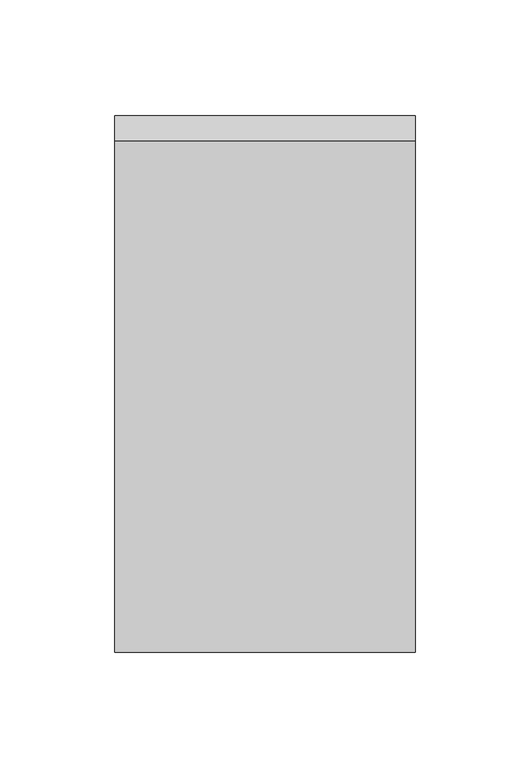
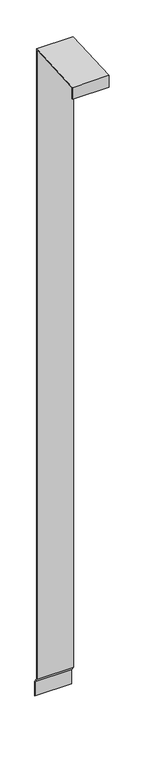
"""IFC4 building model written with IfcOpenShell, lengths in millimetres: proxy geometry, Generic Models 7:Generic Models 1:5:Generic Models 1:5 : Generic Models 7:Generic Models 1:337419:22 : Generic Models 7:Generic Models 1:5:Generic Models 1:5 : Generic Models 7:Generic Models 1:337419:311462."""

from ifc_helpers import new_model, si_unit, frame, origin, place, context, project, spatial, polyline, outline, extrude, source, transform, mapped, element, save


def generic_models_7a759692(model_context):
    return source(origin(), model_context, "Body", "SweptSolid", [
        extrude(outline(polyline([(142.3408058, 0.0), (2525.3911002, 0.0), (2513.9086292, 219.0985972), (2471.5682759, 219.0985972), (2471.5682759, 220.6860972), (2515.4151105, 220.6860972), (2527.0639761, -1.5875), (142.8413427, -1.5875), (126.3142587, -13.1598888), (71.7805947, -13.1598888), (71.7805947, -11.5723888), (125.8137219, -11.5723888), (142.3408058, 0.0)])), frame((560351.7043947, -578783.9976341, 3653.5477111), z_axis=(1.0, -2.1481705303472154e-11, 0.0), x_axis=(0.0, 0.0, 1.0)), (0.0, 0.0, 1.0), 130.6621951),
    ])


if __name__ == "__main__":
    model = new_model("IFC4")
    model_context = context("Model", 3, world=origin())
    ifc_project = project(units=[si_unit("LENGTHUNIT", "METRE", prefix="MILLI")], contexts=[model_context])
    site = spatial("IfcSite", under=ifc_project)
    building = spatial("IfcBuilding", under=site)
    placement = place(None, origin())
    generic_models_shape = generic_models_7a759692(model_context)
    element("IfcBuildingElementProxy", 1, Name="Generic Models 7:Generic Models 1:5:Generic Models 1:5 : Generic Models 7:Generic Models 1:337419:22 : Generic Models 7:Generic Models 1:5:Generic Models 1:5 : Generic Models 7:Generic Models 1:337419:311462", ObjectType="Generic Models 7:Generic Models 1:5:Generic Models 1:5 : Generic Models 7:Generic Models 1:337419:22 : Generic Models 7:Generic Models 1:5:Generic Models 1:5 : Generic Models 7:Generic Models 1:337419:311462", at=placement, inside=building, context=model_context, shape_type="MappedRepresentation", body=[
        mapped(generic_models_shape, transform((0.0, 0.0, 0.0), x_axis=(1.0, 0.0, 0.0), y_axis=(0.0, 1.0, 0.0), z_axis=(0.0, 0.0, 1.0))),
    ])
    save(model, "model.ifc")

# Revit data of these elements
# Type "Generic Models 7:Generic Models 1:5:Generic Models 1:5 : Generic Models 7:Generic Models 1:337419:22 : Generic Models 7:Generic Models 1:5:Generic Models 1:5 : Generic Models 7:Generic Models 1:337419:311462"
#   NameOverride = "Generic Models 7:Generic Models 1:5:Generic Models 1:5 : Generic Models 7:Generic Models 1:337419:311462"
#   ObjectTypeOverride = "Generic Models 1:5 : Generic Models 7:Generic Models 1:337419"
#   Reference = "Generic Models 1"
#   Tag = "311462"
# Element 1 (IfcBuildingElementProxy, "Generic Models 7:Generic Models 1:5:Generic Models 1:5 : Generic Models 7:Generic Models 1:337419:22 : Generic Models 7:Generic Models 1:5:Generic Models 1:5 : Generic Models 7:Generic Models 1:337419:311462")
#   Materials on its faces: "UV STABLE WATER RESISTANT VAPOR PERMEABLE AIR BARRIER (WRB) - WRAP JAMBS/HEADERS - BLACK COLOR"
# Materials
#   "UV STABLE WATER RESISTANT VAPOR PERMEABLE AIR BARRIER (WRB) - WRAP JAMBS/HEADERS - BLACK COLOR": class "Generic", colour RGB 51 162 45, transparency 0, Description = "Polyethylene film membrane", Cost = 0
